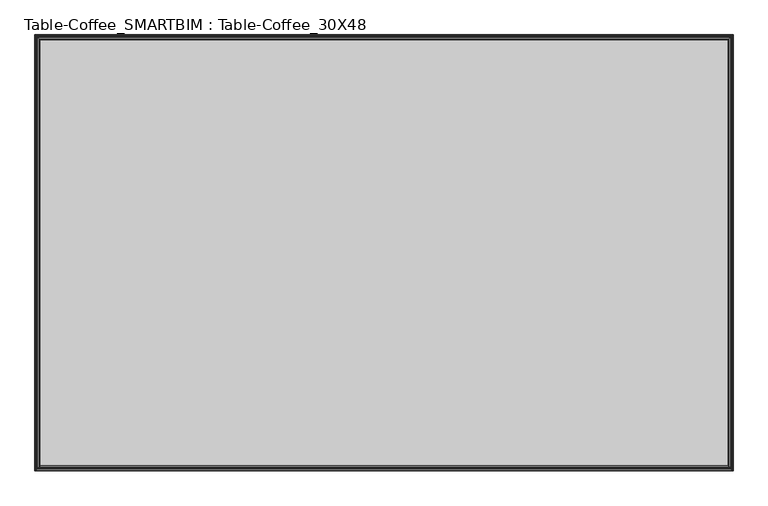
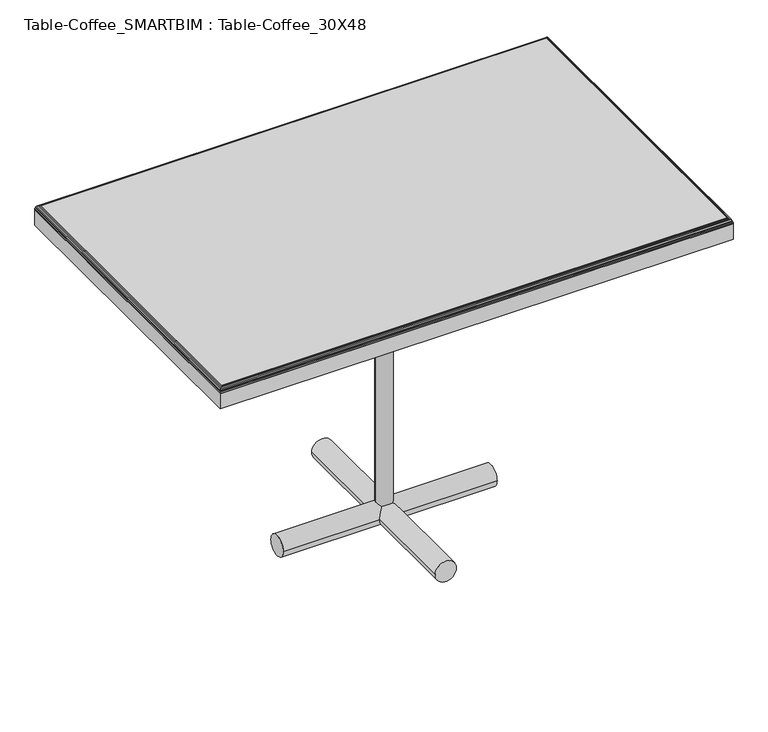
"""IFC4 building model written with IfcOpenShell, lengths in millimetres: furniture geometry, Table-Coffee_SMARTBIM : Table-Coffee_30X48."""

from ifc_helpers import new_model, si_unit, point, frame, frame_2d, origin, origin_2d, place, context, project, spatial, polyline, circle_curve, ellipse_curve, trimmed, segment, composite_curve, outline, extrude, source, transform, mapped, element, save
from ifc_brep_helpers import plane_surface, cylinder_surface, advanced_brep


def table_coffee_smartbim_table_coffee_30x48_01a6e93b(model_context):
    return source(origin(), model_context, "Body", "SolidModel", [
        extrude(outline(composite_curve([segment(trimmed(circle_curve(frame_2d((0.0, 25.4)), 25.4), [point((25.4, 25.4))], [point((-25.4, 25.4))], False, "CARTESIAN"), True, "CONTINUOUS"), segment(trimmed(circle_curve(frame_2d((0.0, 25.4)), 25.4), [point((-25.4, 25.4))], [point((25.4, 25.4))], False, "CARTESIAN"), True, "CONTINUOUS")], self_intersect=False)), frame((-254.0, 0.0, 0.0), z_axis=(1.0, 0.0, 0.0), x_axis=(0.0, 1.0, 0.0)), (0.0, 0.0, 1.0), 508.0),
        extrude(outline(composite_curve([segment(trimmed(circle_curve(frame_2d((25.4, 0.0)), 25.4), [point((25.4, -25.4))], [point((25.4, 25.4))], False, "CARTESIAN"), True, "CONTINUOUS"), segment(trimmed(circle_curve(frame_2d((25.4, 0.0)), 25.4), [point((25.4, 25.4))], [point((25.4, -25.4))], False, "CARTESIAN"), True, "CONTINUOUS")], self_intersect=False)), frame((0.0, -254.0, 0.0), z_axis=(0.0, 1.0, 0.0), x_axis=(0.0, 0.0, 1.0)), (0.0, 0.0, 1.0), 508.0),
        extrude(outline(polyline([(609.6, 381.0), (609.6, -381.0), (-609.6, -381.0), (-609.6, 381.0), (609.6, 381.0)])), frame((0.0, 0.0, 723.9), z_axis=(0.0, 0.0, 1.0), x_axis=(1.0, 0.0, 0.0)), (0.0, 0.0, 1.0), 38.1),
        advanced_brep(
        [(-600.1998654, -371.5998654, 774.7), (600.1998654, -371.5998654, 774.7), (600.1998654, 371.5998654, 774.7), (-600.1998654, 371.5998654, 774.7), (609.6, 381.0, 762.0), (609.6, -381.0, 762.0), (-609.6, -381.0, 762.0), (-609.6, 381.0, 762.0), (-609.6, 381.0, 765.2998654), (609.6, 381.0, 765.2998654), (-609.6, -381.0, 765.2998654), (609.6, -381.0, 765.2998654), (-609.2372483, -380.6372483, 767.8860287), (-609.2372483, 380.6372483, 767.8860287), (-602.3616212, 373.7616212, 774.4480533), (-602.3616212, -373.7616212, 774.4480533), (-604.3639185, 375.7639185, 773.7273912), (-604.3639185, -375.7639185, 773.7273912), (-606.4885738, 377.8885738, 772.2866155), (-606.4885738, -377.8885738, 772.2866155), (-608.5102962, 379.9102962, 769.692959), (-608.5102962, -379.9102962, 769.692959), (609.2372483, -380.6372483, 767.8860287), (602.3616212, -373.7616212, 774.4480533), (604.3639185, -375.7639185, 773.7273912), (606.4885738, -377.8885738, 772.2866155), (608.5102962, -379.9102962, 769.692959), (609.2372483, 380.6372483, 767.8860287), (602.3616212, 373.7616212, 774.4480533), (604.3639185, 375.7639185, 773.7273912), (606.4885738, 377.8885738, 772.2866155), (608.5102962, 379.9102962, 769.692959)],
        [
            (0, 1),
            (1, 2),
            (2, 3),
            (3, 0),
            (4, 5),
            (5, 6),
            (6, 7),
            (7, 4),
            (7, 8),
            (8, 9),
            (9, 4),
            (6, 10),
            (10, 8),
            (5, 11),
            (11, 10),
            (9, 11),
            (10, 12, ellipse_curve(frame((-600.1998654, -371.5998654, 765.2998654), z_axis=(-0.7071067811865475, 0.7071067811865475, 0.0), x_axis=(-0.7071067811865474, -0.7071067811865476, 0.0)), 13.2937978, 9.4001346)),
            (12, 13),
            (13, 8, ellipse_curve(frame((-600.1998654, 371.5998654, 765.2998654), z_axis=(-0.7071067811865475, -0.7071067811865475, 0.0), x_axis=(0.7071067811865474, -0.7071067811865476, 0.0)), 13.2937978, 9.4001346)),
            (14, 15),
            (15, 0, ellipse_curve(frame((-600.1998654, -371.5998654, 765.2998654), z_axis=(-0.7071067811865475, 0.7071067811865475, 0.0), x_axis=(-0.7071067811865474, -0.7071067811865476, 0.0)), 13.2937978, 9.4001346)),
            (3, 14, ellipse_curve(frame((-600.1998654, 371.5998654, 765.2998654), z_axis=(-0.7071067811865475, -0.7071067811865475, 0.0), x_axis=(0.7071067811865474, -0.7071067811865476, 0.0)), 13.2937978, 9.4001346)),
            (14, 16, ellipse_curve(frame((-600.1998654, 371.5998654, 765.2998654), z_axis=(-0.7071067811865475, -0.7071067811865475, 0.0), x_axis=(0.7071067811865474, -0.7071067811865476, 0.0)), 13.2937978, 9.4001346)),
            (16, 17),
            (17, 15, ellipse_curve(frame((-600.1998654, -371.5998654, 765.2998654), z_axis=(-0.7071067811865475, 0.7071067811865475, 0.0), x_axis=(-0.7071067811865474, -0.7071067811865476, 0.0)), 13.2937978, 9.4001346)),
            (16, 18, ellipse_curve(frame((-600.1998654, 371.5998654, 765.2998654), z_axis=(-0.7071067811865475, -0.7071067811865475, 0.0), x_axis=(0.7071067811865474, -0.7071067811865476, 0.0)), 13.2937978, 9.4001346)),
            (18, 19),
            (19, 17, ellipse_curve(frame((-600.1998654, -371.5998654, 765.2998654), z_axis=(-0.7071067811865475, 0.7071067811865475, 0.0), x_axis=(-0.7071067811865474, -0.7071067811865476, 0.0)), 13.2937978, 9.4001346)),
            (18, 20, ellipse_curve(frame((-600.1998654, 371.5998654, 765.2998654), z_axis=(-0.7071067811865475, -0.7071067811865475, 0.0), x_axis=(0.7071067811865474, -0.7071067811865476, 0.0)), 13.2937978, 9.4001346)),
            (20, 21),
            (21, 19, ellipse_curve(frame((-600.1998654, -371.5998654, 765.2998654), z_axis=(-0.7071067811865475, 0.7071067811865475, 0.0), x_axis=(-0.7071067811865474, -0.7071067811865476, 0.0)), 13.2937978, 9.4001346)),
            (12, 21, ellipse_curve(frame((-600.1998654, -371.5998654, 765.2998654), z_axis=(-0.7071067811865475, 0.7071067811865475, 0.0), x_axis=(-0.7071067811865474, -0.7071067811865476, 0.0)), 13.2937978, 9.4001346)),
            (20, 13, ellipse_curve(frame((-600.1998654, 371.5998654, 765.2998654), z_axis=(-0.7071067811865475, -0.7071067811865475, 0.0), x_axis=(0.7071067811865474, -0.7071067811865476, 0.0)), 13.2937978, 9.4001346)),
            (11, 22, ellipse_curve(frame((600.1998654, -371.5998654, 765.2998654), z_axis=(-0.7071067811865475, -0.7071067811865475, 0.0), x_axis=(0.7071067811865476, -0.7071067811865474, 0.0)), 13.2937978, 9.4001346)),
            (22, 12),
            (15, 23),
            (23, 1, ellipse_curve(frame((600.1998654, -371.5998654, 765.2998654), z_axis=(-0.7071067811865475, -0.7071067811865475, 0.0), x_axis=(0.7071067811865476, -0.7071067811865474, 0.0)), 13.2937978, 9.4001346)),
            (17, 24),
            (24, 23, ellipse_curve(frame((600.1998654, -371.5998654, 765.2998654), z_axis=(-0.7071067811865475, -0.7071067811865475, 0.0), x_axis=(0.7071067811865476, -0.7071067811865474, 0.0)), 13.2937978, 9.4001346)),
            (19, 25),
            (25, 24, ellipse_curve(frame((600.1998654, -371.5998654, 765.2998654), z_axis=(-0.7071067811865475, -0.7071067811865475, 0.0), x_axis=(0.7071067811865476, -0.7071067811865474, 0.0)), 13.2937978, 9.4001346)),
            (21, 26),
            (26, 25, ellipse_curve(frame((600.1998654, -371.5998654, 765.2998654), z_axis=(-0.7071067811865475, -0.7071067811865475, 0.0), x_axis=(0.7071067811865476, -0.7071067811865474, 0.0)), 13.2937978, 9.4001346)),
            (22, 26, ellipse_curve(frame((600.1998654, -371.5998654, 765.2998654), z_axis=(-0.7071067811865475, -0.7071067811865475, 0.0), x_axis=(0.7071067811865476, -0.7071067811865474, 0.0)), 13.2937978, 9.4001346)),
            (9, 27, ellipse_curve(frame((600.1998654, 371.5998654, 765.2998654), z_axis=(0.7071067811865475, -0.7071067811865475, 0.0), x_axis=(0.7071067811865474, 0.7071067811865476, 0.0)), 13.2937978, 9.4001346)),
            (27, 22),
            (23, 28),
            (28, 2, ellipse_curve(frame((600.1998654, 371.5998654, 765.2998654), z_axis=(0.7071067811865475, -0.7071067811865475, 0.0), x_axis=(0.7071067811865474, 0.7071067811865476, 0.0)), 13.2937978, 9.4001346)),
            (24, 29),
            (29, 28, ellipse_curve(frame((600.1998654, 371.5998654, 765.2998654), z_axis=(0.7071067811865475, -0.7071067811865475, 0.0), x_axis=(0.7071067811865474, 0.7071067811865476, 0.0)), 13.2937978, 9.4001346)),
            (25, 30),
            (30, 29, ellipse_curve(frame((600.1998654, 371.5998654, 765.2998654), z_axis=(0.7071067811865475, -0.7071067811865475, 0.0), x_axis=(0.7071067811865474, 0.7071067811865476, 0.0)), 13.2937978, 9.4001346)),
            (26, 31),
            (31, 30, ellipse_curve(frame((600.1998654, 371.5998654, 765.2998654), z_axis=(0.7071067811865475, -0.7071067811865475, 0.0), x_axis=(0.7071067811865474, 0.7071067811865476, 0.0)), 13.2937978, 9.4001346)),
            (27, 31, ellipse_curve(frame((600.1998654, 371.5998654, 765.2998654), z_axis=(0.7071067811865475, -0.7071067811865475, 0.0), x_axis=(0.7071067811865474, 0.7071067811865476, 0.0)), 13.2937978, 9.4001346)),
            (13, 27),
            (28, 14),
            (29, 16),
            (30, 18),
            (31, 20),
        ],
        [
            plane_surface(frame((-609.6, 381.0, 774.7), z_axis=(0.0, 0.0, 1.0), x_axis=(-1.0, 0.0, 0.0))),
            plane_surface(frame((-609.6, 381.0, 762.0), z_axis=(0.0, 0.0, -1.0), x_axis=(1.0, 0.0, 0.0))),
            plane_surface(frame((609.6, 381.0, 774.7), z_axis=(0.0, 1.0, 0.0), x_axis=(0.0, 0.0, -1.0))),
            plane_surface(frame((-609.6, 381.0, 774.7), z_axis=(-1.0, 0.0, 0.0), x_axis=(0.0, 0.0, -1.0))),
            plane_surface(frame((-609.6, -381.0, 774.7), z_axis=(0.0, -1.0, 0.0), x_axis=(0.0, 0.0, -1.0))),
            plane_surface(frame((609.6, -381.0, 774.7), z_axis=(1.0, 0.0, 0.0), x_axis=(0.0, 0.0, -1.0))),
            cylinder_surface(frame((-600.1998654, 381.0, 765.2998654), z_axis=(0.0, -1.0, 0.0), x_axis=(1.0, 0.0, 0.0)), 9.4001346),
            cylinder_surface(frame((-609.6, -371.5998654, 765.2998654), z_axis=(1.0, 0.0, 0.0), x_axis=(0.0, 1.0, 0.0)), 9.4001346),
            cylinder_surface(frame((600.1998654, -381.0, 765.2998654), z_axis=(0.0, 1.0, 0.0), x_axis=(-1.0, 0.0, 0.0)), 9.4001346),
            cylinder_surface(frame((609.6, 371.5998654, 765.2998654), z_axis=(-1.0, 0.0, 0.0), x_axis=(0.0, -1.0, 0.0)), 9.4001346),
        ],
        [
            (0, [[1, 2, 3, 4]]),
            (1, [[5, 6, 7, 8]]),
            (2, [[-8, 9, 10, 11]]),
            (3, [[-7, 12, 13, -9]]),
            (4, [[-6, 14, 15, -12]]),
            (5, [[-5, -11, 16, -14]]),
            (6, [[17, 18, 19, -13]]),
            (6, [[20, 21, -4, 22]]),
            (6, [[-20, 23, 24, 25]]),
            (6, [[-24, 26, 27, 28]]),
            (6, [[-27, 29, 30, 31]]),
            (6, [[-18, 32, -30, 33]]),
            (7, [[-17, -15, 34, 35]]),
            (7, [[-21, 36, 37, -1]]),
            (7, [[-25, 38, 39, -36]]),
            (7, [[-28, 40, 41, -38]]),
            (7, [[-31, 42, 43, -40]]),
            (7, [[-32, -35, 44, -42]]),
            (8, [[-34, -16, 45, 46]]),
            (8, [[-37, 47, 48, -2]]),
            (8, [[-39, 49, 50, -47]]),
            (8, [[-41, 51, 52, -49]]),
            (8, [[-43, 53, 54, -51]]),
            (8, [[-44, -46, 55, -53]]),
            (9, [[-19, 56, -45, -10]]),
            (9, [[-22, -3, -48, 57]]),
            (9, [[-23, -57, -50, 58]]),
            (9, [[-26, -58, -52, 59]]),
            (9, [[-29, -59, -54, 60]]),
            (9, [[-33, -60, -55, -56]]),
        ],
    ),
        extrude(outline(polyline([(76.2, 76.2), (76.2, -76.2), (-76.2, -76.2), (-76.2, 76.2), (76.2, 76.2)])), frame((0.0, 0.0, 755.65), z_axis=(0.0, 0.0, 1.0), x_axis=(1.0, 0.0, 0.0)), (0.0, 0.0, 1.0), 6.35),
        extrude(outline(composite_curve([segment(trimmed(circle_curve(origin_2d(), 19.05), [point((-19.05, 0.0))], [point((19.05, 0.0))], False, "CARTESIAN"), True, "CONTINUOUS"), segment(trimmed(circle_curve(origin_2d(), 19.05), [point((19.05, 0.0))], [point((-19.05, 0.0))], False, "CARTESIAN"), True, "CONTINUOUS")], self_intersect=False)), frame((0.0, 0.0, 24.2070278), z_axis=(0.0, 0.0, 1.0), x_axis=(1.0, 0.0, 0.0)), (0.0, 0.0, 1.0), 731.4429722),
    ])


if __name__ == "__main__":
    model = new_model("IFC4")
    model_context = context("Model", 3, world=origin())
    ifc_project = project(units=[si_unit("LENGTHUNIT", "METRE", prefix="MILLI")], contexts=[model_context])
    site = spatial("IfcSite", under=ifc_project)
    building = spatial("IfcBuilding", under=site)
    placement = place(None, origin())
    table_coffee_smartbim_table_coffee_30x48_shape = table_coffee_smartbim_table_coffee_30x48_01a6e93b(model_context)
    element("IfcFurniture", 1, ObjectType="Table-Coffee_SMARTBIM : Table-Coffee_30X48", at=placement, inside=building, context=model_context, shape_type="MappedRepresentation", body=[
        mapped(table_coffee_smartbim_table_coffee_30x48_shape, transform((0.0, 0.0, 0.0), x_axis=(1.0, 0.0, 0.0), y_axis=(0.0, 1.0, 0.0), z_axis=(0.0, 0.0, 1.0))),
    ])
    save(model, "model.ifc")

# Revit data of these elements
# Type "Table-Coffee_SMARTBIM : Table-Coffee_30X48"
#   Subcategory = "Table\r\n"
#   SmartBIM Object Created By = "SMARTBIM, LLC"
#   Manufacturer = "SMARTBIM"
#   Assembly Code = "E2020200"
#   95 CSI = "12500"
#   04 CSI = "12 50 00"
#   table cloth = 0' - 1 1/2"
#   Width = 4' - 0"
#   SmartBIM Object Version = 3
#   Height = 2' - 6"
#   Depth = 2' - 6"
#   Default Elevation = 4' - 0"
#   white cloth_parameter = Sals Wood
#   Table Unit = MET
#   Glide = none
#   Glass = none
# Element 1 (IfcFurniture, "Table-Coffee_SMARTBIM : Table-Coffee_30X48")
#   Materials on its faces: "Sals Wood", "MET"
# Materials
#   "Sals Wood": class "Wood", colour RGB 198 202 183, transparency 0, Description = "Generic wood", Cost = 0
#   "MET": class "Metal", colour RGB 189 187 185, transparency 0
